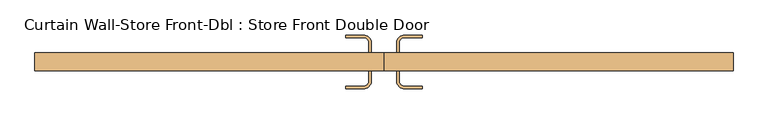
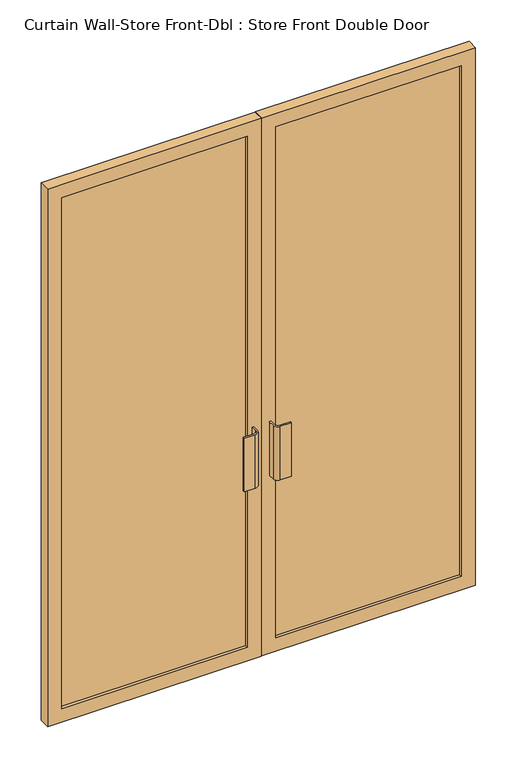
"""IFC4 building model written with IfcOpenShell, lengths in millimetres: door geometry, Curtain Wall-Store Front-Dbl : Store Front Double Door."""

import ifcopenshell
import ifcopenshell.guid

model = None  # the IFC model being written
_history = None  # IfcOwnerHistory: only IFC2X3 demands one
_inside = {}  # id of a spatial element -> (the spatial element, [elements in it])
_under = {}  # id of a project, library or spatial element -> (it, [spatial elements below it])
_declared = {}  # id of a project -> (the project, [libraries it declares])
_typed = {}  # id of a type object -> (the type object, [elements of that type])
_made_of = {}  # id of a material, layer set ... -> (it, [elements and type objects made of it])


def new_model(schema):
    """Start an empty IFC model of exactly this schema.

    Asked for "IFC4X3", IfcOpenShell would pick the latest addendum, in which some entities
    have other attributes; the version numbers below select the first issue.
    IFC2X3 requires an IfcOwnerHistory on every rooted entity: one is made here for all.
    """
    global model, _history
    if schema == "IFC4X3":
        model = ifcopenshell.file(schema_version=(4, 3, 0, 0))
    else:
        model = ifcopenshell.file(schema=schema)
    _inside.clear()
    _under.clear()
    _declared.clear()
    _typed.clear()
    _made_of.clear()
    _history = None
    if model.schema == "IFC2X3":
        org = make("IfcOrganization", Name="unknown")
        user = make(
            "IfcPersonAndOrganization",
            ThePerson=make("IfcPerson", FamilyName="unknown"),
            TheOrganization=org,
        )
        app = make(
            "IfcApplication",
            ApplicationDeveloper=org,
            Version="unknown",
            ApplicationFullName="unknown",
            ApplicationIdentifier="unknown",
        )
        _history = make(
            "IfcOwnerHistory",
            OwningUser=user,
            OwningApplication=app,
            ChangeAction="ADDED",
            CreationDate=0,
        )
    return model


def make(cls, **values):
    """One entity of the class cls with the attributes given. An attribute that is None is left unset."""
    return model.create_entity(
        cls, **{name: value for name, value in values.items() if value is not None}
    )


def rooted(cls, **values):
    """An entity with a GlobalId (a new one), such as an element, a storey or a relation."""
    return make(cls, GlobalId=ifcopenshell.guid.new(), OwnerHistory=_history, **values)


def si_unit(unit_type, name, prefix=None):
    """IfcSIUnit, for example si_unit("LENGTHUNIT", "METRE", prefix="MILLI")."""
    return make("IfcSIUnit", UnitType=unit_type, Prefix=prefix, Name=name)


def assignment(units):
    """IfcUnitAssignment: the units of a project."""
    return None if units is None else make("IfcUnitAssignment", Units=units)


def point(xyz):
    """IfcCartesianPoint."""
    return None if xyz is None else make("IfcCartesianPoint", Coordinates=xyz)


def direction(xyz):
    """IfcDirection."""
    return None if xyz is None else make("IfcDirection", DirectionRatios=xyz)


def frame(location, z_axis=None, x_axis=None):
    """IfcAxis2Placement3D, a coordinate frame: its origin and axes. An axis left out is left unset."""
    return make(
        "IfcAxis2Placement3D",
        Location=point(location),
        Axis=direction(z_axis),
        RefDirection=direction(x_axis),
    )


def frame_2d(location, x_axis=None):
    """IfcAxis2Placement2D, a coordinate frame in the plane: its origin and x axis."""
    return make(
        "IfcAxis2Placement2D", Location=point(location), RefDirection=direction(x_axis)
    )


def origin():
    """The frame at (0, 0, 0) with its axes left unset."""
    return frame((0.0, 0.0, 0.0))


def place(relative_to, where):
    """IfcLocalPlacement: puts the frame where relative to a parent placement (None: the world)."""
    return make(
        "IfcLocalPlacement", PlacementRelTo=relative_to, RelativePlacement=where
    )


def context(
    kind, dimensions, precision=None, world=None, true_north=None, identifier=None
):
    """IfcGeometricRepresentationContext, for example the 3D "Model" context."""
    return make(
        "IfcGeometricRepresentationContext",
        ContextIdentifier=identifier,
        ContextType=kind,
        CoordinateSpaceDimension=dimensions,
        Precision=precision,
        WorldCoordinateSystem=world,
        TrueNorth=true_north,
    )


def project(units=None, contexts=None):
    """IfcProject with its units and contexts."""
    return rooted(
        "IfcProject",
        Name="project",
        RepresentationContexts=contexts,
        UnitsInContext=assignment(units),
    )


def spatial(cls, under=None, at=None, **own):
    """A site, building, storey or space (cls), placed at a placement, below another one or the project."""
    s = rooted(cls, ObjectPlacement=at, **own)
    if under is not None:
        _under.setdefault(under.id(), (under, []))[1].append(s)
    return s


def polyline(points):
    """IfcPolyline through the points."""
    return make("IfcPolyline", Points=[point(p) for p in points])


def circle_curve(where, radius):
    """IfcCircle in the frame where."""
    return make("IfcCircle", Position=where, Radius=radius)


def trimmed(basis, trim1, trim2, sense, master):
    """IfcTrimmedCurve: the piece of a basis curve between two trims."""
    return make(
        "IfcTrimmedCurve",
        BasisCurve=basis,
        Trim1=trim1,
        Trim2=trim2,
        SenseAgreement=sense,
        MasterRepresentation=master,
    )


def segment(curve, same_sense, transition):
    """IfcCompositeCurveSegment."""
    return make(
        "IfcCompositeCurveSegment",
        Transition=transition,
        SameSense=same_sense,
        ParentCurve=curve,
    )


def composite_curve(segments, self_intersect=None):
    """IfcCompositeCurve: segments joined end to end."""
    return make("IfcCompositeCurve", Segments=segments, SelfIntersect=self_intersect)


def outline(outer, holes=None, kind="AREA"):
    """IfcArbitraryClosedProfileDef: a profile drawn as a closed curve; with holes, ...WithVoids."""
    if holes is None:
        return make("IfcArbitraryClosedProfileDef", ProfileType=kind, OuterCurve=outer)
    return make(
        "IfcArbitraryProfileDefWithVoids",
        ProfileType=kind,
        OuterCurve=outer,
        InnerCurves=holes,
    )


def extrude(swept, where, along, depth):
    """IfcExtrudedAreaSolid: the profile swept, set in the frame where, extruded along a direction by depth."""
    return make(
        "IfcExtrudedAreaSolid",
        SweptArea=swept,
        Position=where,
        ExtrudedDirection=direction(along),
        Depth=depth,
    )


def shape(context_of_items, identifier, shape_type, items):
    """IfcShapeRepresentation: the items that make up one representation, for example the "Body"."""
    return make(
        "IfcShapeRepresentation",
        ContextOfItems=context_of_items,
        RepresentationIdentifier=identifier,
        RepresentationType=shape_type,
        Items=items,
    )


def source(mapping_origin, context_of_items, identifier, shape_type, items):
    """IfcRepresentationMap: a shape defined once, which mapped items show again and again."""
    return make(
        "IfcRepresentationMap",
        MappingOrigin=mapping_origin,
        MappedRepresentation=shape(context_of_items, identifier, shape_type, items),
    )


def transform(
    local_origin,
    x_axis=None,
    y_axis=None,
    z_axis=None,
    scale=None,
    scale2=None,
    scale3=None,
    uniform=True,
):
    """IfcCartesianTransformationOperator3D, or its non-uniform kind. x_axis, y_axis, z_axis: its Axis1, 2, 3."""
    if uniform:
        return make(
            "IfcCartesianTransformationOperator3D",
            Axis1=direction(x_axis),
            Axis2=direction(y_axis),
            LocalOrigin=point(local_origin),
            Scale=scale,
            Axis3=direction(z_axis),
        )
    return make(
        "IfcCartesianTransformationOperator3DnonUniform",
        Axis1=direction(x_axis),
        Axis2=direction(y_axis),
        LocalOrigin=point(local_origin),
        Scale=scale,
        Axis3=direction(z_axis),
        Scale2=scale2,
        Scale3=scale3,
    )


def mapped(mapping_source, mapping_target):
    """IfcMappedItem: shows the shape of a source again, moved by a transform."""
    return make(
        "IfcMappedItem", MappingSource=mapping_source, MappingTarget=mapping_target
    )


def made_of(thing, what):
    """Note that an element or type object is made of a material, layer set ...; save() writes the relation."""
    if what is not None:
        _made_of.setdefault(what.id(), (what, []))[1].append(thing)
    return thing


def element(
    cls,
    number,
    at=None,
    inside=None,
    cuts=None,
    type_object=None,
    material=None,
    context=None,
    identifier="Body",
    shape_type=None,
    held_by="IfcProductDefinitionShape",
    body=None,
    shapes=None,
    **own,
):
    """One element of the class cls, such as IfcWall. Its Tag is "e" and its number.

    at: its placement. inside: the storey or other place that contains it. cuts: it is an
    opening in that element (IfcRelVoidsElement). A single representation is given by context,
    identifier, shape_type and body (its items); several are given by shapes. held_by: the class
    of the entity that holds the representations. save() writes the other relations.
    """
    e = rooted(cls, Tag="e%d" % number, ObjectPlacement=at, **own)
    if body is not None:
        shapes = [shape(context, identifier, shape_type, body)]
    if shapes is not None:
        e.Representation = make(held_by, Representations=shapes)
    if inside is not None:
        _inside.setdefault(inside.id(), (inside, []))[1].append(e)
    if cuts is not None:
        rooted(
            "IfcRelVoidsElement", RelatingBuildingElement=cuts, RelatedOpeningElement=e
        )
    if type_object is not None:
        _typed.setdefault(type_object.id(), (type_object, []))[1].append(e)
    return made_of(e, material)


def aggregate(whole, parts):
    """IfcRelAggregates: a whole, such as a stair, and the parts it consists of."""
    return rooted("IfcRelAggregates", RelatingObject=whole, RelatedObjects=parts)


def save(model, path):
    """Write the relations noted so far, then the file.

    IfcRelAggregates (storeys below a building ...), IfcRelContainedInSpatialStructure (elements
    in a storey), IfcRelDefinesByType, IfcRelAssociatesMaterial and IfcRelDeclares: one each for
    every whole, place, type object, material and project.
    """
    for whole, parts in _under.values():
        aggregate(whole, parts)
    for where, things in _inside.values():
        rooted(
            "IfcRelContainedInSpatialStructure",
            RelatedElements=things,
            RelatingStructure=where,
        )
    for kind, things in _typed.values():
        rooted("IfcRelDefinesByType", RelatedObjects=things, RelatingType=kind)
    for what, things in _made_of.values():
        rooted("IfcRelAssociatesMaterial", RelatedObjects=things, RelatingMaterial=what)
    for by, libraries in _declared.values():
        rooted("IfcRelDeclares", RelatingContext=by, RelatedDefinitions=libraries)
    model.write(path)


def curtain_wall_store_front_dbl_store_front_double_door_239a7903(model_context):
    return source(origin(), model_context, "Body", "SweptSolid", [
        extrude(outline(composite_curve([segment(polyline([(-31.75, 12.7), (-31.75, -12.7), (-38.1, -12.7), (-38.1, 12.7)]), True, "CONTINUOUS"), segment(trimmed(circle_curve(frame_2d((-50.8, 12.7)), 12.7), [point((-38.1, 12.7))], [point((-50.8, 25.4))], True, "CARTESIAN"), True, "CONTINUOUS"), segment(polyline([(-50.8, 25.4), (-95.25, 25.4), (-95.25, 31.75), (-50.8, 31.75)]), True, "CONTINUOUS"), segment(trimmed(circle_curve(frame_2d((-50.8, 12.7)), 19.05), [point((-50.8, 31.75))], [point((-31.75, 12.7))], False, "CARTESIAN"), True, "CONTINUOUS")], self_intersect=False)), frame((0.0, 0.0, 762.0), z_axis=(0.0, 0.0, 1.0), x_axis=(1.0, 0.0, 0.0)), (0.0, 0.0, 1.0), 228.6),
        extrude(outline(composite_curve([segment(trimmed(circle_curve(frame_2d((50.8, 12.7)), 19.05), [point((31.75, 12.7))], [point((50.8, 31.75))], False, "CARTESIAN"), True, "CONTINUOUS"), segment(polyline([(50.8, 31.75), (95.25, 31.75), (95.25, 25.4), (50.8, 25.4)]), True, "CONTINUOUS"), segment(trimmed(circle_curve(frame_2d((50.8, 12.7)), 12.7), [point((50.8, 25.4))], [point((38.1, 12.7))], True, "CARTESIAN"), True, "CONTINUOUS"), segment(polyline([(38.1, 12.7), (38.1, -12.7), (31.75, -12.7), (31.75, 12.7)]), True, "CONTINUOUS")], self_intersect=False)), frame((0.0, 0.0, 762.0), z_axis=(0.0, 0.0, 1.0), x_axis=(1.0, 0.0, 0.0)), (0.0, 0.0, 1.0), 228.6),
        extrude(outline(composite_curve([segment(trimmed(circle_curve(frame_2d((-50.8, -82.55)), 19.05), [point((-31.75, -82.55))], [point((-50.8, -101.6))], False, "CARTESIAN"), True, "CONTINUOUS"), segment(polyline([(-50.8, -101.6), (-95.25, -101.6), (-95.25, -95.25), (-50.8, -95.25)]), True, "CONTINUOUS"), segment(trimmed(circle_curve(frame_2d((-50.8, -82.55)), 12.7), [point((-50.8, -95.25))], [point((-38.1, -82.55))], True, "CARTESIAN"), True, "CONTINUOUS"), segment(polyline([(-38.1, -82.55), (-38.1, -57.15), (-31.75, -57.15), (-31.75, -82.55)]), True, "CONTINUOUS")], self_intersect=False)), frame((0.0, 0.0, 762.0), z_axis=(0.0, 0.0, 1.0), x_axis=(1.0, 0.0, 0.0)), (0.0, 0.0, 1.0), 228.6),
        extrude(outline(composite_curve([segment(polyline([(31.75, -82.55), (31.75, -57.15), (38.1, -57.15), (38.1, -82.55)]), True, "CONTINUOUS"), segment(trimmed(circle_curve(frame_2d((50.8, -82.55)), 12.7), [point((38.1, -82.55))], [point((50.8, -95.25))], True, "CARTESIAN"), True, "CONTINUOUS"), segment(polyline([(50.8, -95.25), (95.25, -95.25), (95.25, -101.6), (50.8, -101.6)]), True, "CONTINUOUS"), segment(trimmed(circle_curve(frame_2d((50.8, -82.55)), 19.05), [point((50.8, -101.6))], [point((31.75, -82.55))], False, "CARTESIAN"), True, "CONTINUOUS")], self_intersect=False)), frame((0.0, 0.0, 762.0), z_axis=(0.0, 0.0, 1.0), x_axis=(1.0, 0.0, 0.0)), (0.0, 0.0, 1.0), 228.6),
        extrude(outline(polyline([(807.4671284, -25.4), (807.4671284, -44.45), (57.94375, -44.45), (57.94375, -25.4), (807.4671284, -25.4)])), frame((0.0, 0.0, 57.15), z_axis=(0.0, 0.0, 1.0), x_axis=(1.0, 0.0, 0.0)), (0.0, 0.0, 1.0), 2182.8125),
        extrude(outline(polyline([(-57.94375, -25.4), (-57.94375, -44.45), (-807.4671284, -44.45), (-807.4671284, -25.4), (-57.94375, -25.4)])), frame((0.0, 0.0, 57.15), z_axis=(0.0, 0.0, 1.0), x_axis=(1.0, 0.0, 0.0)), (0.0, 0.0, 1.0), 2182.8125),
        extrude(outline(polyline([(2297.1125, 0.79375), (0.0, 0.79375), (0.0, 864.6171284), (2297.1125, 864.6171284), (2297.1125, 0.79375)]), holes=[polyline([(2239.9625, 57.94375), (2239.9625, 807.4671284), (57.15, 807.4671284), (57.15, 57.94375), (2239.9625, 57.94375)])]), frame((0.0, -57.15, 0.0), z_axis=(0.0, 1.0, 0.0), x_axis=(0.0, 0.0, 1.0)), (0.0, 0.0, 1.0), 44.45),
        extrude(outline(polyline([(2297.1125, -0.79375), (2297.1125, -864.6171284), (0.0, -864.6171284), (0.0, -0.79375), (2297.1125, -0.79375)]), holes=[polyline([(2239.9625, -807.4671284), (2239.9625, -57.94375), (57.15, -57.94375), (57.15, -807.4671284), (2239.9625, -807.4671284)])]), frame((0.0, -57.15, 0.0), z_axis=(0.0, 1.0, 0.0), x_axis=(0.0, 0.0, 1.0)), (0.0, 0.0, 1.0), 44.45),
    ])


if __name__ == "__main__":
    model = new_model("IFC4")
    model_context = context("Model", 3, world=origin())
    ifc_project = project(units=[si_unit("LENGTHUNIT", "METRE", prefix="MILLI")], contexts=[model_context])
    site = spatial("IfcSite", under=ifc_project)
    building = spatial("IfcBuilding", under=site)
    placement = place(None, origin())
    curtain_wall_store_front_dbl_store_front_double_door_shape = curtain_wall_store_front_dbl_store_front_double_door_239a7903(model_context)
    element("IfcDoor", 1, ObjectType="Curtain Wall-Store Front-Dbl : Store Front Double Door", at=placement, inside=building, context=model_context, shape_type="MappedRepresentation", body=[
        mapped(curtain_wall_store_front_dbl_store_front_double_door_shape, transform((0.0, 0.0, 0.0), x_axis=(1.0, 0.0, 0.0), y_axis=(0.0, 1.0, 0.0), z_axis=(0.0, 0.0, 1.0))),
    ])
    save(model, "model.ifc")

# Revit data of these elements
# Type "Curtain Wall-Store Front-Dbl : Store Front Double Door"
#   Type Mark = "17"
#   Construction Type Id = "MDOOR"
#   Assembly Code = "B2030110"
#   Analytic Construction = "Metal"
#   Offset = 0' - 2 1/4"
#   Heat Transfer Coefficient (U) = 3.7021 W/(m²·K)
#   Function = 1
#   Material = Aluminum
#   Glazing Material = Glass
#   Visual Light Transmittance = 0
#   Solar Heat Gain Coefficient = 0
# Element 1 (IfcDoor, "Curtain Wall-Store Front-Dbl : Store Front Double Door")
#   Materials on its faces: "Aluminum", "Glass"
# Materials
#   "Aluminum": class "Metal", colour RGB 247 247 247, transparency 0, Description = "Aluminum 6061", Cost = 0
#   "Glass": class "Unassigned", colour RGB 0 0 255, transparency 0.75
